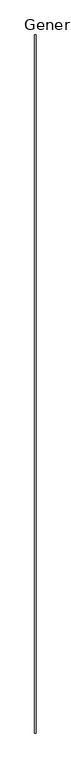
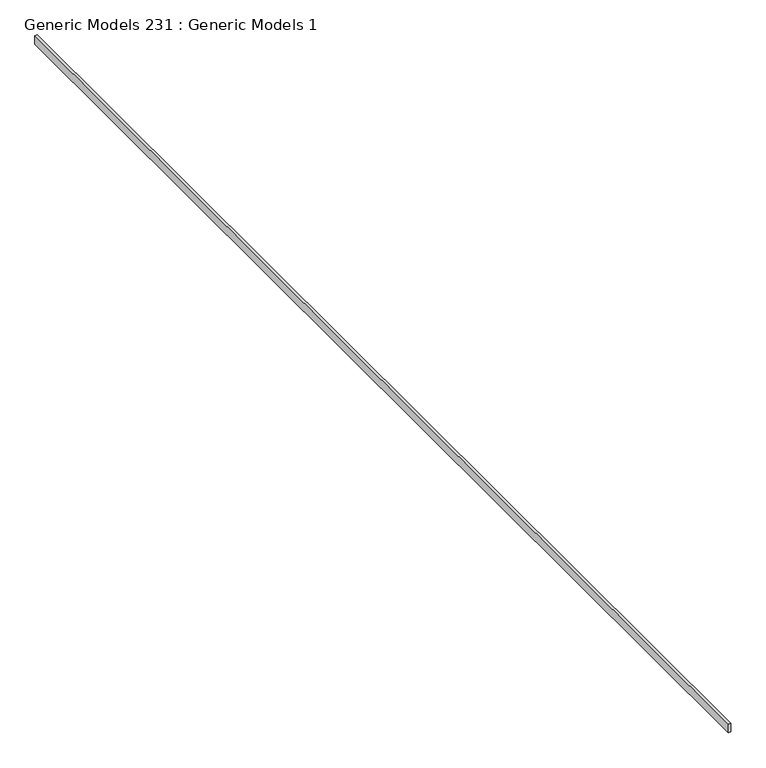
"""IFC4 building model written with IfcOpenShell, lengths in millimetres: proxy geometry, Generic Models 231 : Generic Models 1."""

import ifcopenshell
import ifcopenshell.guid

model = None  # the IFC model being written
_history = None  # IfcOwnerHistory: only IFC2X3 demands one
_inside = {}  # id of a spatial element -> (the spatial element, [elements in it])
_under = {}  # id of a project, library or spatial element -> (it, [spatial elements below it])
_declared = {}  # id of a project -> (the project, [libraries it declares])
_typed = {}  # id of a type object -> (the type object, [elements of that type])
_made_of = {}  # id of a material, layer set ... -> (it, [elements and type objects made of it])


def new_model(schema):
    """Start an empty IFC model of exactly this schema.

    Asked for "IFC4X3", IfcOpenShell would pick the latest addendum, in which some entities
    have other attributes; the version numbers below select the first issue.
    IFC2X3 requires an IfcOwnerHistory on every rooted entity: one is made here for all.
    """
    global model, _history
    if schema == "IFC4X3":
        model = ifcopenshell.file(schema_version=(4, 3, 0, 0))
    else:
        model = ifcopenshell.file(schema=schema)
    _inside.clear()
    _under.clear()
    _declared.clear()
    _typed.clear()
    _made_of.clear()
    _history = None
    if model.schema == "IFC2X3":
        org = make("IfcOrganization", Name="unknown")
        user = make(
            "IfcPersonAndOrganization",
            ThePerson=make("IfcPerson", FamilyName="unknown"),
            TheOrganization=org,
        )
        app = make(
            "IfcApplication",
            ApplicationDeveloper=org,
            Version="unknown",
            ApplicationFullName="unknown",
            ApplicationIdentifier="unknown",
        )
        _history = make(
            "IfcOwnerHistory",
            OwningUser=user,
            OwningApplication=app,
            ChangeAction="ADDED",
            CreationDate=0,
        )
    return model


def make(cls, **values):
    """One entity of the class cls with the attributes given. An attribute that is None is left unset."""
    return model.create_entity(
        cls, **{name: value for name, value in values.items() if value is not None}
    )


def rooted(cls, **values):
    """An entity with a GlobalId (a new one), such as an element, a storey or a relation."""
    return make(cls, GlobalId=ifcopenshell.guid.new(), OwnerHistory=_history, **values)


def si_unit(unit_type, name, prefix=None):
    """IfcSIUnit, for example si_unit("LENGTHUNIT", "METRE", prefix="MILLI")."""
    return make("IfcSIUnit", UnitType=unit_type, Prefix=prefix, Name=name)


def assignment(units):
    """IfcUnitAssignment: the units of a project."""
    return None if units is None else make("IfcUnitAssignment", Units=units)


def point(xyz):
    """IfcCartesianPoint."""
    return None if xyz is None else make("IfcCartesianPoint", Coordinates=xyz)


def direction(xyz):
    """IfcDirection."""
    return None if xyz is None else make("IfcDirection", DirectionRatios=xyz)


def frame(location, z_axis=None, x_axis=None):
    """IfcAxis2Placement3D, a coordinate frame: its origin and axes. An axis left out is left unset."""
    return make(
        "IfcAxis2Placement3D",
        Location=point(location),
        Axis=direction(z_axis),
        RefDirection=direction(x_axis),
    )


def origin():
    """The frame at (0, 0, 0) with its axes left unset."""
    return frame((0.0, 0.0, 0.0))


def place(relative_to, where):
    """IfcLocalPlacement: puts the frame where relative to a parent placement (None: the world)."""
    return make(
        "IfcLocalPlacement", PlacementRelTo=relative_to, RelativePlacement=where
    )


def context(
    kind, dimensions, precision=None, world=None, true_north=None, identifier=None
):
    """IfcGeometricRepresentationContext, for example the 3D "Model" context."""
    return make(
        "IfcGeometricRepresentationContext",
        ContextIdentifier=identifier,
        ContextType=kind,
        CoordinateSpaceDimension=dimensions,
        Precision=precision,
        WorldCoordinateSystem=world,
        TrueNorth=true_north,
    )


def project(units=None, contexts=None):
    """IfcProject with its units and contexts."""
    return rooted(
        "IfcProject",
        Name="project",
        RepresentationContexts=contexts,
        UnitsInContext=assignment(units),
    )


def spatial(cls, under=None, at=None, **own):
    """A site, building, storey or space (cls), placed at a placement, below another one or the project."""
    s = rooted(cls, ObjectPlacement=at, **own)
    if under is not None:
        _under.setdefault(under.id(), (under, []))[1].append(s)
    return s


def polyline(points):
    """IfcPolyline through the points."""
    return make("IfcPolyline", Points=[point(p) for p in points])


def outline(outer, holes=None, kind="AREA"):
    """IfcArbitraryClosedProfileDef: a profile drawn as a closed curve; with holes, ...WithVoids."""
    if holes is None:
        return make("IfcArbitraryClosedProfileDef", ProfileType=kind, OuterCurve=outer)
    return make(
        "IfcArbitraryProfileDefWithVoids",
        ProfileType=kind,
        OuterCurve=outer,
        InnerCurves=holes,
    )


def extrude(swept, where, along, depth):
    """IfcExtrudedAreaSolid: the profile swept, set in the frame where, extruded along a direction by depth."""
    return make(
        "IfcExtrudedAreaSolid",
        SweptArea=swept,
        Position=where,
        ExtrudedDirection=direction(along),
        Depth=depth,
    )


def shape(context_of_items, identifier, shape_type, items):
    """IfcShapeRepresentation: the items that make up one representation, for example the "Body"."""
    return make(
        "IfcShapeRepresentation",
        ContextOfItems=context_of_items,
        RepresentationIdentifier=identifier,
        RepresentationType=shape_type,
        Items=items,
    )


def source(mapping_origin, context_of_items, identifier, shape_type, items):
    """IfcRepresentationMap: a shape defined once, which mapped items show again and again."""
    return make(
        "IfcRepresentationMap",
        MappingOrigin=mapping_origin,
        MappedRepresentation=shape(context_of_items, identifier, shape_type, items),
    )


def transform(
    local_origin,
    x_axis=None,
    y_axis=None,
    z_axis=None,
    scale=None,
    scale2=None,
    scale3=None,
    uniform=True,
):
    """IfcCartesianTransformationOperator3D, or its non-uniform kind. x_axis, y_axis, z_axis: its Axis1, 2, 3."""
    if uniform:
        return make(
            "IfcCartesianTransformationOperator3D",
            Axis1=direction(x_axis),
            Axis2=direction(y_axis),
            LocalOrigin=point(local_origin),
            Scale=scale,
            Axis3=direction(z_axis),
        )
    return make(
        "IfcCartesianTransformationOperator3DnonUniform",
        Axis1=direction(x_axis),
        Axis2=direction(y_axis),
        LocalOrigin=point(local_origin),
        Scale=scale,
        Axis3=direction(z_axis),
        Scale2=scale2,
        Scale3=scale3,
    )


def mapped(mapping_source, mapping_target):
    """IfcMappedItem: shows the shape of a source again, moved by a transform."""
    return make(
        "IfcMappedItem", MappingSource=mapping_source, MappingTarget=mapping_target
    )


def made_of(thing, what):
    """Note that an element or type object is made of a material, layer set ...; save() writes the relation."""
    if what is not None:
        _made_of.setdefault(what.id(), (what, []))[1].append(thing)
    return thing


def element(
    cls,
    number,
    at=None,
    inside=None,
    cuts=None,
    type_object=None,
    material=None,
    context=None,
    identifier="Body",
    shape_type=None,
    held_by="IfcProductDefinitionShape",
    body=None,
    shapes=None,
    **own,
):
    """One element of the class cls, such as IfcWall. Its Tag is "e" and its number.

    at: its placement. inside: the storey or other place that contains it. cuts: it is an
    opening in that element (IfcRelVoidsElement). A single representation is given by context,
    identifier, shape_type and body (its items); several are given by shapes. held_by: the class
    of the entity that holds the representations. save() writes the other relations.
    """
    e = rooted(cls, Tag="e%d" % number, ObjectPlacement=at, **own)
    if body is not None:
        shapes = [shape(context, identifier, shape_type, body)]
    if shapes is not None:
        e.Representation = make(held_by, Representations=shapes)
    if inside is not None:
        _inside.setdefault(inside.id(), (inside, []))[1].append(e)
    if cuts is not None:
        rooted(
            "IfcRelVoidsElement", RelatingBuildingElement=cuts, RelatedOpeningElement=e
        )
    if type_object is not None:
        _typed.setdefault(type_object.id(), (type_object, []))[1].append(e)
    return made_of(e, material)


def aggregate(whole, parts):
    """IfcRelAggregates: a whole, such as a stair, and the parts it consists of."""
    return rooted("IfcRelAggregates", RelatingObject=whole, RelatedObjects=parts)


def save(model, path):
    """Write the relations noted so far, then the file.

    IfcRelAggregates (storeys below a building ...), IfcRelContainedInSpatialStructure (elements
    in a storey), IfcRelDefinesByType, IfcRelAssociatesMaterial and IfcRelDeclares: one each for
    every whole, place, type object, material and project.
    """
    for whole, parts in _under.values():
        aggregate(whole, parts)
    for where, things in _inside.values():
        rooted(
            "IfcRelContainedInSpatialStructure",
            RelatedElements=things,
            RelatingStructure=where,
        )
    for kind, things in _typed.values():
        rooted("IfcRelDefinesByType", RelatedObjects=things, RelatingType=kind)
    for what, things in _made_of.values():
        rooted("IfcRelAssociatesMaterial", RelatedObjects=things, RelatingMaterial=what)
    for by, libraries in _declared.values():
        rooted("IfcRelDeclares", RelatingContext=by, RelatedDefinitions=libraries)
    model.write(path)


def generic_models_231_generic_models_1_a16331ab(model_context):
    return source(origin(), model_context, "Body", "SweptSolid", [
        extrude(outline(polyline([(1580.9763704, 11981.8769662), (1619.0763704, 11981.8769662), (1619.0763704, -7068.1230338), (1580.9763704, -7068.1230338), (1580.9763704, 11981.8769662)])), frame((0.0, 0.0, 126263.146), z_axis=(0.0, 0.0, 1.0), x_axis=(1.0, 0.0, 0.0)), (0.0, 0.0, 1.0), 139.7),
    ])


if __name__ == "__main__":
    model = new_model("IFC4")
    model_context = context("Model", 3, world=origin())
    ifc_project = project(units=[si_unit("LENGTHUNIT", "METRE", prefix="MILLI")], contexts=[model_context])
    site = spatial("IfcSite", under=ifc_project)
    building = spatial("IfcBuilding", under=site)
    placement = place(None, origin())
    generic_models_231_generic_models_1_shape = generic_models_231_generic_models_1_a16331ab(model_context)
    element("IfcBuildingElementProxy", 1, Name="Generic Models 231 : Generic Models 1", ObjectType="Generic Models 231 : Generic Models 1", at=placement, inside=building, context=model_context, shape_type="MappedRepresentation", body=[
        mapped(generic_models_231_generic_models_1_shape, transform((0.0, 0.0, 0.0), x_axis=(1.0, 0.0, 0.0), y_axis=(0.0, 1.0, 0.0), z_axis=(0.0, 0.0, 1.0))),
    ])
    save(model, "model.ifc")

# Revit data of these elements
# Element 1 (IfcBuildingElementProxy, "Generic Models 231 : Generic Models 1")
#   Materials on its faces: "_STRUCTURAL MEMBER (SEE STRUCT. DWGS)"
# Materials
#   "_STRUCTURAL MEMBER (SEE STRUCT. DWGS)": class "Generic", colour RGB 209 182 141, transparency 0, Cost = 0
